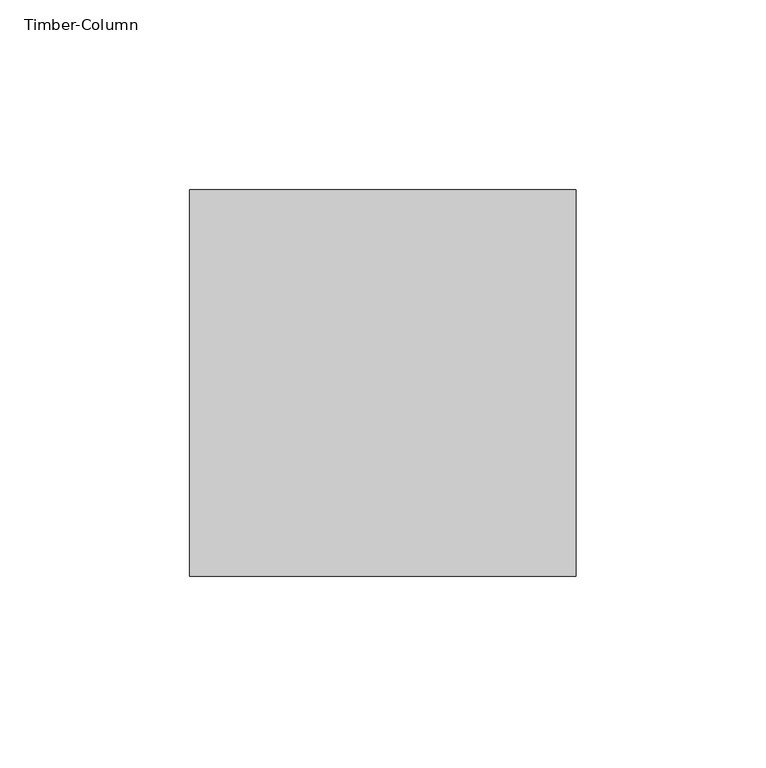
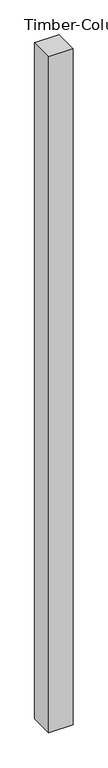
"""IFC4 building model written with IfcOpenShell, lengths in millimetres: column geometry, Timber-Column."""

from ifc_helpers import new_model, si_unit, frame, origin, place, context, project, spatial, polyline, outline, extrude, source, transform, mapped, element, save


def timber_column_8a3ad47c(model_context):
    return source(origin(), model_context, "Body", "SweptSolid", [
        extrude(outline(polyline([(50.8, 50.8), (50.8, -50.8), (-50.8, -50.8), (-50.8, 50.8), (50.8, 50.8)])), frame((0.0, 0.0, -319.88125), z_axis=(0.0, 0.0, 1.0), x_axis=(1.0, 0.0, 0.0)), (0.0, 0.0, 1.0), 2986.88125),
    ])


if __name__ == "__main__":
    model = new_model("IFC4")
    model_context = context("Model", 3, world=origin())
    ifc_project = project(units=[si_unit("LENGTHUNIT", "METRE", prefix="MILLI")], contexts=[model_context])
    site = spatial("IfcSite", under=ifc_project)
    building = spatial("IfcBuilding", under=site)
    placement = place(None, origin())
    timber_column_shape = timber_column_8a3ad47c(model_context)
    element("IfcColumn", 1, ObjectType="Timber-Column : BLDG 6241 Wall Struds 4\"x4\"", at=placement, inside=building, context=model_context, shape_type="MappedRepresentation", body=[
        mapped(timber_column_shape, transform((0.0, 0.0, 0.0), x_axis=(1.0, 0.0, 0.0), y_axis=(0.0, 1.0, 0.0), z_axis=(0.0, 0.0, 1.0))),
    ])
    save(model, "model.ifc")

# Revit data of these elements
# Type "Timber-Column : BLDG 6241 Wall Struds 4\"x4\""
#   Assembly Code = "B10"
#   A = 0.140625 SF
#   b = 0' - 4"
#   d = 0' - 4"
#   Structural Material [instance default] = Softwood, Lumber
# Element 1 (IfcColumn, "Timber-Column : BLDG 6241 Wall Struds 4\"x4\"")
#   Materials on its faces: "Softwood, Lumber"
# Materials
#   "Softwood, Lumber": class "Wood", colour RGB 223 192 134, transparency 0, Description = "Pinus Echinata", Cost = 0
